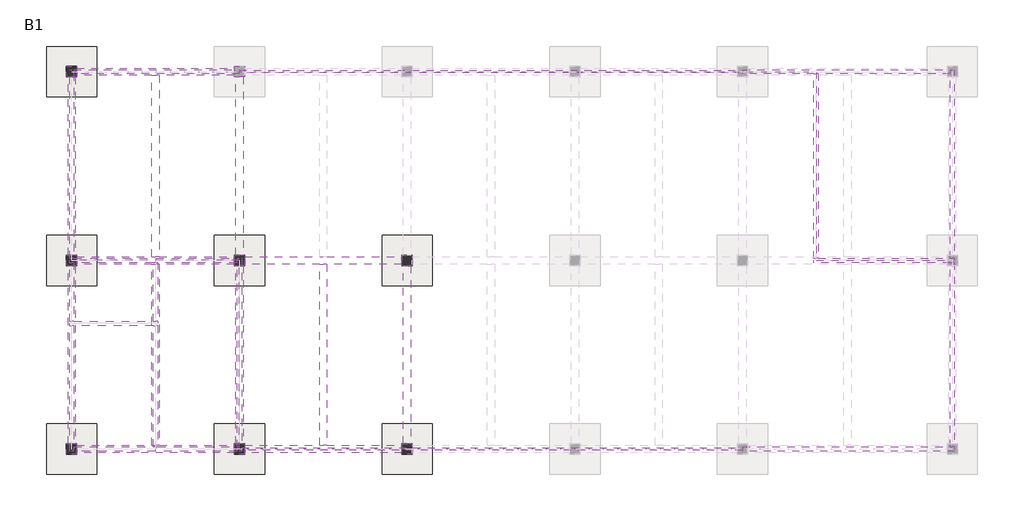
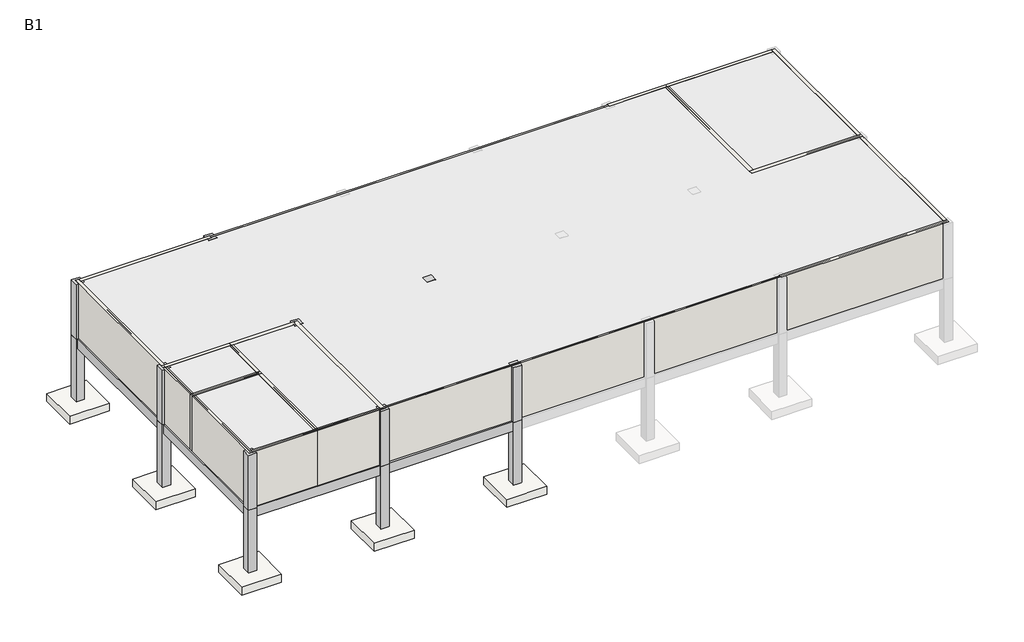
# One storey, part 1 of 2: 20 walls, 15 columns, 13 beams, 12 slabs.
"""IFC4 building model written with IfcOpenShell, lengths in millimetres."""

import ifcopenshell
import ifcopenshell.guid

model = None  # the IFC model being written
_history = None  # IfcOwnerHistory: only IFC2X3 demands one
_inside = {}  # id of a spatial element -> (the spatial element, [elements in it])
_under = {}  # id of a project, library or spatial element -> (it, [spatial elements below it])
_declared = {}  # id of a project -> (the project, [libraries it declares])
_typed = {}  # id of a type object -> (the type object, [elements of that type])
_made_of = {}  # id of a material, layer set ... -> (it, [elements and type objects made of it])


def new_model(schema):
    """Start an empty IFC model of exactly this schema.

    Asked for "IFC4X3", IfcOpenShell would pick the latest addendum, in which some entities
    have other attributes; the version numbers below select the first issue.
    IFC2X3 requires an IfcOwnerHistory on every rooted entity: one is made here for all.
    """
    global model, _history
    if schema == "IFC4X3":
        model = ifcopenshell.file(schema_version=(4, 3, 0, 0))
    else:
        model = ifcopenshell.file(schema=schema)
    _inside.clear()
    _under.clear()
    _declared.clear()
    _typed.clear()
    _made_of.clear()
    _history = None
    if model.schema == "IFC2X3":
        org = make("IfcOrganization", Name="unknown")
        user = make(
            "IfcPersonAndOrganization",
            ThePerson=make("IfcPerson", FamilyName="unknown"),
            TheOrganization=org,
        )
        app = make(
            "IfcApplication",
            ApplicationDeveloper=org,
            Version="unknown",
            ApplicationFullName="unknown",
            ApplicationIdentifier="unknown",
        )
        _history = make(
            "IfcOwnerHistory",
            OwningUser=user,
            OwningApplication=app,
            ChangeAction="ADDED",
            CreationDate=0,
        )
    return model


def make(cls, **values):
    """One entity of the class cls with the attributes given. An attribute that is None is left unset."""
    return model.create_entity(
        cls, **{name: value for name, value in values.items() if value is not None}
    )


def rooted(cls, **values):
    """An entity with a GlobalId (a new one), such as an element, a storey or a relation."""
    return make(cls, GlobalId=ifcopenshell.guid.new(), OwnerHistory=_history, **values)


def si_unit(unit_type, name, prefix=None):
    """IfcSIUnit, for example si_unit("LENGTHUNIT", "METRE", prefix="MILLI")."""
    return make("IfcSIUnit", UnitType=unit_type, Prefix=prefix, Name=name)


def assignment(units):
    """IfcUnitAssignment: the units of a project."""
    return None if units is None else make("IfcUnitAssignment", Units=units)


def point(xyz):
    """IfcCartesianPoint."""
    return None if xyz is None else make("IfcCartesianPoint", Coordinates=xyz)


def direction(xyz):
    """IfcDirection."""
    return None if xyz is None else make("IfcDirection", DirectionRatios=xyz)


def frame(location, z_axis=None, x_axis=None):
    """IfcAxis2Placement3D, a coordinate frame: its origin and axes. An axis left out is left unset."""
    return make(
        "IfcAxis2Placement3D",
        Location=point(location),
        Axis=direction(z_axis),
        RefDirection=direction(x_axis),
    )


def origin():
    """The frame at (0, 0, 0) with its axes left unset."""
    return frame((0.0, 0.0, 0.0))


def origin_with_axes():
    """The frame at (0, 0, 0) with the z axis (0, 0, 1) and the x axis (1, 0, 0) written out."""
    return frame((0.0, 0.0, 0.0), z_axis=(0.0, 0.0, 1.0), x_axis=(1.0, 0.0, 0.0))


def place(relative_to, where):
    """IfcLocalPlacement: puts the frame where relative to a parent placement (None: the world)."""
    return make(
        "IfcLocalPlacement", PlacementRelTo=relative_to, RelativePlacement=where
    )


def context(
    kind, dimensions, precision=None, world=None, true_north=None, identifier=None
):
    """IfcGeometricRepresentationContext, for example the 3D "Model" context."""
    return make(
        "IfcGeometricRepresentationContext",
        ContextIdentifier=identifier,
        ContextType=kind,
        CoordinateSpaceDimension=dimensions,
        Precision=precision,
        WorldCoordinateSystem=world,
        TrueNorth=true_north,
    )


def project(units=None, contexts=None):
    """IfcProject with its units and contexts."""
    return rooted(
        "IfcProject",
        Name="project",
        RepresentationContexts=contexts,
        UnitsInContext=assignment(units),
    )


def spatial(cls, under=None, at=None, **own):
    """A site, building, storey or space (cls), placed at a placement, below another one or the project."""
    s = rooted(cls, ObjectPlacement=at, **own)
    if under is not None:
        _under.setdefault(under.id(), (under, []))[1].append(s)
    return s


def polyline(points):
    """IfcPolyline through the points."""
    return make("IfcPolyline", Points=[point(p) for p in points])


def outline(outer, holes=None, kind="AREA"):
    """IfcArbitraryClosedProfileDef: a profile drawn as a closed curve; with holes, ...WithVoids."""
    if holes is None:
        return make("IfcArbitraryClosedProfileDef", ProfileType=kind, OuterCurve=outer)
    return make(
        "IfcArbitraryProfileDefWithVoids",
        ProfileType=kind,
        OuterCurve=outer,
        InnerCurves=holes,
    )


def extrude(swept, where, along, depth):
    """IfcExtrudedAreaSolid: the profile swept, set in the frame where, extruded along a direction by depth."""
    return make(
        "IfcExtrudedAreaSolid",
        SweptArea=swept,
        Position=where,
        ExtrudedDirection=direction(along),
        Depth=depth,
    )


def faces_of(points, faces, orient=None, outer=None):
    """IfcFace entities. A face is a list of loops; a loop is a list of indices into points, from 0.

    orient and outer hold one flag for each loop. By default every Orientation is true, the
    first loop of a face is its IfcFaceOuterBound and the others are IfcFaceBound.
    """
    made = []
    for i, loops in enumerate(faces):
        bounds = []
        for j, loop in enumerate(loops):
            is_outer = j == 0 if outer is None else outer[i][j]
            bounds.append(
                make(
                    "IfcFaceOuterBound" if is_outer else "IfcFaceBound",
                    Bound=make("IfcPolyLoop", Polygon=[points[k] for k in loop]),
                    Orientation=True if orient is None else orient[i][j],
                )
            )
        made.append(make("IfcFace", Bounds=bounds))
    return made


def faceted_brep(points, faces, orient=None, outer=None, voids=None):
    """IfcFacetedBrep: a solid bounded by flat faces; with voids (closed shells), ...WithVoids."""
    shared = [point(p) for p in points]
    hull = make("IfcClosedShell", CfsFaces=faces_of(shared, faces, orient, outer))
    if voids is None:
        return make("IfcFacetedBrep", Outer=hull)
    return make(
        "IfcFacetedBrepWithVoids",
        Outer=hull,
        Voids=[
            make(cls, CfsFaces=faces_of(shared, fs, o, b)) for cls, fs, o, b in voids
        ],
    )


def shape(context_of_items, identifier, shape_type, items):
    """IfcShapeRepresentation: the items that make up one representation, for example the "Body"."""
    return make(
        "IfcShapeRepresentation",
        ContextOfItems=context_of_items,
        RepresentationIdentifier=identifier,
        RepresentationType=shape_type,
        Items=items,
    )


def source(mapping_origin, context_of_items, identifier, shape_type, items):
    """IfcRepresentationMap: a shape defined once, which mapped items show again and again."""
    return make(
        "IfcRepresentationMap",
        MappingOrigin=mapping_origin,
        MappedRepresentation=shape(context_of_items, identifier, shape_type, items),
    )


def transform(
    local_origin,
    x_axis=None,
    y_axis=None,
    z_axis=None,
    scale=None,
    scale2=None,
    scale3=None,
    uniform=True,
):
    """IfcCartesianTransformationOperator3D, or its non-uniform kind. x_axis, y_axis, z_axis: its Axis1, 2, 3."""
    if uniform:
        return make(
            "IfcCartesianTransformationOperator3D",
            Axis1=direction(x_axis),
            Axis2=direction(y_axis),
            LocalOrigin=point(local_origin),
            Scale=scale,
            Axis3=direction(z_axis),
        )
    return make(
        "IfcCartesianTransformationOperator3DnonUniform",
        Axis1=direction(x_axis),
        Axis2=direction(y_axis),
        LocalOrigin=point(local_origin),
        Scale=scale,
        Axis3=direction(z_axis),
        Scale2=scale2,
        Scale3=scale3,
    )


def mapped(mapping_source, mapping_target):
    """IfcMappedItem: shows the shape of a source again, moved by a transform."""
    return make(
        "IfcMappedItem", MappingSource=mapping_source, MappingTarget=mapping_target
    )


def made_of(thing, what):
    """Note that an element or type object is made of a material, layer set ...; save() writes the relation."""
    if what is not None:
        _made_of.setdefault(what.id(), (what, []))[1].append(thing)
    return thing


def element(
    cls,
    number,
    at=None,
    inside=None,
    cuts=None,
    type_object=None,
    material=None,
    context=None,
    identifier="Body",
    shape_type=None,
    held_by="IfcProductDefinitionShape",
    body=None,
    shapes=None,
    **own,
):
    """One element of the class cls, such as IfcWall. Its Tag is "e" and its number.

    at: its placement. inside: the storey or other place that contains it. cuts: it is an
    opening in that element (IfcRelVoidsElement). A single representation is given by context,
    identifier, shape_type and body (its items); several are given by shapes. held_by: the class
    of the entity that holds the representations. save() writes the other relations.
    """
    e = rooted(cls, Tag="e%d" % number, ObjectPlacement=at, **own)
    if body is not None:
        shapes = [shape(context, identifier, shape_type, body)]
    if shapes is not None:
        e.Representation = make(held_by, Representations=shapes)
    if inside is not None:
        _inside.setdefault(inside.id(), (inside, []))[1].append(e)
    if cuts is not None:
        rooted(
            "IfcRelVoidsElement", RelatingBuildingElement=cuts, RelatedOpeningElement=e
        )
    if type_object is not None:
        _typed.setdefault(type_object.id(), (type_object, []))[1].append(e)
    return made_of(e, material)


def aggregate(whole, parts):
    """IfcRelAggregates: a whole, such as a stair, and the parts it consists of."""
    return rooted("IfcRelAggregates", RelatingObject=whole, RelatedObjects=parts)


def save(model, path):
    """Write the relations noted so far, then the file.

    IfcRelAggregates (storeys below a building ...), IfcRelContainedInSpatialStructure (elements
    in a storey), IfcRelDefinesByType, IfcRelAssociatesMaterial and IfcRelDeclares: one each for
    every whole, place, type object, material and project.
    """
    for whole, parts in _under.values():
        aggregate(whole, parts)
    for where, things in _inside.values():
        rooted(
            "IfcRelContainedInSpatialStructure",
            RelatedElements=things,
            RelatingStructure=where,
        )
    for kind, things in _typed.values():
        rooted("IfcRelDefinesByType", RelatedObjects=things, RelatingType=kind)
    for what, things in _made_of.values():
        rooted("IfcRelAssociatesMaterial", RelatedObjects=things, RelatingMaterial=what)
    for by, libraries in _declared.values():
        rooted("IfcRelDeclares", RelatingContext=by, RelatedDefinitions=libraries)
    model.write(path)


def ft112_footing_rectangular_ft112_2400x2400x500_5fe39465(model_context):
    return source(origin(), model_context, "Body", "SweptSolid", [
        extrude(outline(polyline([(1200.0, 1200.0), (1200.0, -1200.0), (-1200.0, -1200.0), (-1200.0, 1200.0), (1200.0, 1200.0)])), frame((0.0, 0.0, -500.0), z_axis=(0.0, 0.0, 1.0), x_axis=(1.0, 0.0, 0.0)), (0.0, 0.0, 1.0), 500.0),
    ])


model = new_model("IFC4")

# Units and contexts
model_context = context("Model", 3, world=origin())
ifc_project = project(units=[si_unit("LENGTHUNIT", "METRE", prefix="MILLI")], contexts=[model_context])

# Site, building, storey
site = spatial("IfcSite", under=ifc_project)
building = spatial("IfcBuilding", under=site)
storey = spatial("IfcBuildingStorey", under=building, Name="B1", Elevation=-4000.0)

# Beams
placement = place(None, origin())
element("IfcBeam", 1, ObjectType="Concrete-Rectangular-Beam : BM111_400x500_RG1", at=placement, inside=storey, context=model_context, shape_type="SweptSolid", body=[
    extrude(outline(polyline([(49284.6521483, 181748.8614395), (49634.6521483, 181748.8614395), (49634.6521483, 173098.8614395), (49284.6521483, 173098.8614395), (49284.6521483, 181748.8614395)])), frame((0.0, 0.0, -600.0), z_axis=(0.0, 0.0, 1.0), x_axis=(1.0, 0.0, 0.0)), (0.0, 0.0, 1.0), 600.0),
])
element("IfcBeam", 2, ObjectType="Concrete-Rectangular-Beam : BM111_400x500_RG1", at=placement, inside=storey, context=model_context, shape_type="SweptSolid", body=[
    extrude(outline(polyline([(49284.6521483, 172748.8614395), (49634.6521483, 172748.8614395), (49634.6521483, 164098.8614395), (49284.6521483, 164098.8614395), (49284.6521483, 172748.8614395)])), frame((0.0, 0.0, -600.0), z_axis=(0.0, 0.0, 1.0), x_axis=(1.0, 0.0, 0.0)), (0.0, 0.0, 1.0), 600.0),
])
element("IfcBeam", 3, ObjectType="Concrete-Rectangular-Beam : BM111_400x500_RG1", at=placement, inside=storey, context=model_context, shape_type="SweptSolid", body=[
    extrude(outline(polyline([(57284.6521483, 172748.8614395), (57634.6521483, 172748.8614395), (57634.6521483, 164098.8614395), (57284.6521483, 164098.8614395), (57284.6521483, 172748.8614395)])), frame((0.0, 0.0, -600.0), z_axis=(0.0, 0.0, 1.0), x_axis=(1.0, 0.0, 0.0)), (0.0, 0.0, 1.0), 600.0),
])
element("IfcBeam", 4, ObjectType="Concrete-Rectangular-Beam : BM111_400x500_RG1", at=placement, inside=storey, context=model_context, shape_type="Brep", body=[
    faceted_brep([(45709.6521483, 182098.8614395, 0.0), (45709.6521483, 181748.8614395, 0.0), (49284.6521483, 181748.8614395, 0.0), (49634.6521483, 181748.8614395, 0.0), (53209.6521483, 181748.8614395, 0.0), (53209.6521483, 182098.8614395, 0.0), (45709.6521483, 181748.8614395, -600.0), (49284.6521483, 181748.8614395, -600.0), (49634.6521483, 181748.8614395, -600.0), (53209.6521483, 181748.8614395, -600.0), (45709.6521483, 182098.8614395, -600.0), (53209.6521483, 182098.8614395, -600.0)], [[[0, 1, 2, 3, 4, 5]], [[1, 6, 7, 8, 9, 4, 3, 2]], [[6, 10, 11, 9, 8, 7]], [[10, 0, 5, 11]], [[1, 0, 10, 6]], [[5, 4, 9, 11]]]),
])
element("IfcBeam", 5, ObjectType="Concrete-Rectangular-Beam : BM111_400x500_RG1", at=placement, inside=storey, context=model_context, shape_type="Brep", body=[
    faceted_brep([(45709.6521483, 173098.8614395, 0.0), (45709.6521483, 172748.8614395, 0.0), (49284.6521483, 172748.8614395, 0.0), (49634.6521483, 172748.8614395, 0.0), (53209.6521483, 172748.8614395, 0.0), (53209.6521483, 173098.8614395, 0.0), (49634.6521483, 173098.8614395, 0.0), (49284.6521483, 173098.8614395, 0.0), (45709.6521483, 172748.8614395, -600.0), (49284.6521483, 172748.8614395, -600.0), (49634.6521483, 172748.8614395, -600.0), (53209.6521483, 172748.8614395, -600.0), (45709.6521483, 173098.8614395, -600.0), (49284.6521483, 173098.8614395, -600.0), (49634.6521483, 173098.8614395, -600.0), (53209.6521483, 173098.8614395, -600.0)], [[[0, 1, 2, 3, 4, 5, 6, 7]], [[1, 8, 9, 10, 11, 4, 3, 2]], [[8, 12, 13, 14, 15, 11, 10, 9]], [[12, 0, 7, 6, 5, 15, 14, 13]], [[1, 0, 12, 8]], [[5, 4, 11, 15]]]),
])
element("IfcBeam", 6, ObjectType="Concrete-Rectangular-Beam : BM111_400x500_RG1", at=placement, inside=storey, context=model_context, shape_type="Brep", body=[
    faceted_brep([(53709.6521483, 173098.8614395, 0.0), (53709.6521483, 172748.8614395, 0.0), (57284.6521483, 172748.8614395, 0.0), (57634.6521483, 172748.8614395, 0.0), (61209.6521483, 172748.8614395, 0.0), (61209.6521483, 173098.8614395, 0.0), (57634.6521483, 173098.8614395, 0.0), (57284.6521483, 173098.8614395, 0.0), (53709.6521483, 172748.8614395, -600.0), (57284.6521483, 172748.8614395, -600.0), (57634.6521483, 172748.8614395, -600.0), (61209.6521483, 172748.8614395, -600.0), (53709.6521483, 173098.8614395, -600.0), (57284.6521483, 173098.8614395, -600.0), (57634.6521483, 173098.8614395, -600.0), (61209.6521483, 173098.8614395, -600.0)], [[[0, 1, 2, 3, 4, 5, 6, 7]], [[1, 8, 9, 10, 11, 4, 3, 2]], [[8, 12, 13, 14, 15, 11, 10, 9]], [[12, 0, 7, 6, 5, 15, 14, 13]], [[1, 0, 12, 8]], [[5, 4, 11, 15]]]),
])
element("IfcBeam", 7, ObjectType="Concrete-Rectangular-Beam : BM111_400x500_RG1", at=placement, inside=storey, context=model_context, shape_type="Brep", body=[
    faceted_brep([(45709.6521483, 164098.8614395, 0.0), (45709.6521483, 163748.8614395, 0.0), (53209.6521483, 163748.8614395, 0.0), (53209.6521483, 164098.8614395, 0.0), (49634.6521483, 164098.8614395, 0.0), (49284.6521483, 164098.8614395, 0.0), (45709.6521483, 163748.8614395, -600.0), (53209.6521483, 163748.8614395, -600.0), (45709.6521483, 164098.8614395, -600.0), (49284.6521483, 164098.8614395, -600.0), (49634.6521483, 164098.8614395, -600.0), (53209.6521483, 164098.8614395, -600.0)], [[[0, 1, 2, 3, 4, 5]], [[1, 6, 7, 2]], [[6, 8, 9, 10, 11, 7]], [[8, 0, 5, 4, 3, 11, 10, 9]], [[1, 0, 8, 6]], [[3, 2, 7, 11]]]),
])
element("IfcBeam", 8, ObjectType="Concrete-Rectangular-Beam : BM111_400x500_RG1", at=placement, inside=storey, context=model_context, shape_type="Brep", body=[
    faceted_brep([(53709.6521483, 164098.8614395, 0.0), (53709.6521483, 163748.8614395, 0.0), (61209.6521483, 163748.8614395, 0.0), (61209.6521483, 164098.8614395, 0.0), (57634.6521483, 164098.8614395, 0.0), (57284.6521483, 164098.8614395, 0.0), (53709.6521483, 163748.8614395, -600.0), (61209.6521483, 163748.8614395, -600.0), (53709.6521483, 164098.8614395, -600.0), (57284.6521483, 164098.8614395, -600.0), (57634.6521483, 164098.8614395, -600.0), (61209.6521483, 164098.8614395, -600.0)], [[[0, 1, 2, 3, 4, 5]], [[1, 6, 7, 2]], [[6, 8, 9, 10, 11, 7]], [[8, 0, 5, 4, 3, 11, 10, 9]], [[1, 0, 8, 6]], [[3, 2, 7, 11]]]),
])
element("IfcBeam", 9, ObjectType="Concrete-Rectangular-Beam : BM111_400x500_RG1", at=placement, inside=storey, context=model_context, shape_type="SweptSolid", body=[
    extrude(outline(polyline([(45284.6521483, 181673.8614395), (45634.6521483, 181673.8614395), (45634.6521483, 173173.8614395), (45284.6521483, 173173.8614395), (45284.6521483, 181673.8614395)])), frame((0.0, 0.0, -600.0), z_axis=(0.0, 0.0, 1.0), x_axis=(1.0, 0.0, 0.0)), (0.0, 0.0, 1.0), 600.0),
])
element("IfcBeam", 10, ObjectType="Concrete-Rectangular-Beam : BM111_400x500_RG1", at=placement, inside=storey, context=model_context, shape_type="SweptSolid", body=[
    extrude(outline(polyline([(45284.6521483, 172673.8614395), (45634.6521483, 172673.8614395), (45634.6521483, 164173.8614395), (45284.6521483, 164173.8614395), (45284.6521483, 172673.8614395)])), frame((0.0, 0.0, -600.0), z_axis=(0.0, 0.0, 1.0), x_axis=(1.0, 0.0, 0.0)), (0.0, 0.0, 1.0), 600.0),
])
element("IfcBeam", 11, ObjectType="Concrete-Rectangular-Beam : BM111_400x500_RG1", at=placement, inside=storey, context=model_context, shape_type="SweptSolid", body=[
    extrude(outline(polyline([(53284.6521483, 181673.8614395), (53634.6521483, 181673.8614395), (53634.6521483, 173173.8614395), (53284.6521483, 173173.8614395), (53284.6521483, 181673.8614395)])), frame((0.0, 0.0, -600.0), z_axis=(0.0, 0.0, 1.0), x_axis=(1.0, 0.0, 0.0)), (0.0, 0.0, 1.0), 600.0),
])
element("IfcBeam", 12, ObjectType="Concrete-Rectangular-Beam : BM111_400x500_RG1", at=placement, inside=storey, context=model_context, shape_type="SweptSolid", body=[
    extrude(outline(polyline([(53284.6521483, 172673.8614395), (53634.6521483, 172673.8614395), (53634.6521483, 164173.8614395), (53284.6521483, 164173.8614395), (53284.6521483, 172673.8614395)])), frame((0.0, 0.0, -600.0), z_axis=(0.0, 0.0, 1.0), x_axis=(1.0, 0.0, 0.0)), (0.0, 0.0, 1.0), 600.0),
])
element("IfcBeam", 13, ObjectType="Concrete-Rectangular-Beam : BM111_400x500_RG1", at=placement, inside=storey, context=model_context, shape_type="SweptSolid", body=[
    extrude(outline(polyline([(61284.6521483, 172673.8614395), (61634.6521483, 172673.8614395), (61634.6521483, 164173.8614395), (61284.6521483, 164173.8614395), (61284.6521483, 172673.8614395)])), frame((0.0, 0.0, -600.0), z_axis=(0.0, 0.0, 1.0), x_axis=(1.0, 0.0, 0.0)), (0.0, 0.0, 1.0), 600.0),
])

# Columns
element("IfcColumn", 14, ObjectType="Concrete-Rectangular-Column : CL111_500x500", at=placement, inside=storey, context=model_context, shape_type="Brep", body=[
    faceted_brep([(45709.6521483, 182173.8614395, 0.0), (45709.6521483, 181673.8614395, 0.0), (45209.6521483, 181673.8614395, 0.0), (45209.6521483, 182173.8614395, 0.0), (45709.6521483, 182173.8614395, 3500.0), (45709.6521483, 182098.8614395, 3500.0), (45709.6521483, 181748.8614395, 3500.0), (45709.6521483, 181673.8614395, 3500.0), (45634.6521483, 181673.8614395, 3500.0), (45284.6521483, 181673.8614395, 3500.0), (45209.6521483, 181673.8614395, 3500.0), (45209.6521483, 182173.8614395, 3500.0)], [[[0, 1, 2, 3]], [[4, 5, 6, 7, 1, 0]], [[7, 8, 9, 10, 2, 1]], [[10, 11, 3, 2]], [[11, 4, 0, 3]], [[4, 11, 10, 9, 8, 7, 6, 5]]]),
])
element("IfcColumn", 15, ObjectType="Concrete-Rectangular-Column : CL111_500x500", at=placement, inside=storey, context=model_context, shape_type="Brep", body=[
    faceted_brep([(53709.6521483, 182173.8614395, 0.0), (53709.6521483, 181673.8614395, 0.0), (53209.6521483, 181673.8614395, 0.0), (53209.6521483, 182173.8614395, 0.0), (53709.6521483, 182173.8614395, 3500.0), (53709.6521483, 182098.8614395, 3500.0), (53709.6521483, 181748.8614395, 3500.0), (53709.6521483, 181673.8614395, 3500.0), (53634.6521483, 181673.8614395, 3500.0), (53284.6521483, 181673.8614395, 3500.0), (53209.6521483, 181673.8614395, 3500.0), (53209.6521483, 181748.8614395, 3500.0), (53209.6521483, 182098.8614395, 3500.0), (53209.6521483, 182173.8614395, 3500.0)], [[[0, 1, 2, 3]], [[4, 5, 6, 7, 1, 0]], [[7, 8, 9, 10, 2, 1]], [[10, 11, 12, 13, 3, 2]], [[13, 4, 0, 3]], [[4, 13, 12, 11, 10, 9, 8, 7, 6, 5]]]),
])
element("IfcColumn", 16, ObjectType="Concrete-Rectangular-Column : CL111_500x500", at=placement, inside=storey, context=model_context, shape_type="Brep", body=[
    faceted_brep([(45709.6521483, 173173.8614395, 0.0), (45709.6521483, 172673.8614395, 0.0), (45209.6521483, 172673.8614395, 0.0), (45209.6521483, 173173.8614395, 0.0), (45709.6521483, 173173.8614395, 3500.0), (45709.6521483, 173098.8614395, 3500.0), (45709.6521483, 172748.8614395, 3500.0), (45709.6521483, 172673.8614395, 3500.0), (45634.6521483, 172673.8614395, 3500.0), (45284.6521483, 172673.8614395, 3500.0), (45209.6521483, 172673.8614395, 3500.0), (45209.6521483, 173173.8614395, 3500.0), (45284.6521483, 173173.8614395, 3500.0), (45634.6521483, 173173.8614395, 3500.0)], [[[0, 1, 2, 3]], [[4, 5, 6, 7, 1, 0]], [[7, 8, 9, 10, 2, 1]], [[10, 11, 3, 2]], [[11, 12, 13, 4, 0, 3]], [[4, 13, 12, 11, 10, 9, 8, 7, 6, 5]]]),
])
element("IfcColumn", 17, ObjectType="Concrete-Rectangular-Column : CL111_500x500", at=placement, inside=storey, context=model_context, shape_type="Brep", body=[
    faceted_brep([(53709.6521483, 173173.8614395, 0.0), (53709.6521483, 172673.8614395, 0.0), (53209.6521483, 172673.8614395, 0.0), (53209.6521483, 173173.8614395, 0.0), (53709.6521483, 173173.8614395, 3500.0), (53709.6521483, 173098.8614395, 3500.0), (53709.6521483, 172748.8614395, 3500.0), (53709.6521483, 172673.8614395, 3500.0), (53634.6521483, 172673.8614395, 3500.0), (53284.6521483, 172673.8614395, 3500.0), (53209.6521483, 172673.8614395, 3500.0), (53209.6521483, 172748.8614395, 3500.0), (53209.6521483, 173098.8614395, 3500.0), (53209.6521483, 173173.8614395, 3500.0), (53284.6521483, 173173.8614395, 3500.0), (53634.6521483, 173173.8614395, 3500.0)], [[[0, 1, 2, 3]], [[4, 5, 6, 7, 1, 0]], [[7, 8, 9, 10, 2, 1]], [[10, 11, 12, 13, 3, 2]], [[13, 14, 15, 4, 0, 3]], [[4, 15, 14, 13, 12, 11, 10, 9, 8, 7, 6, 5]]]),
])
element("IfcColumn", 18, ObjectType="Concrete-Rectangular-Column : CL111_500x500", at=placement, inside=storey, context=model_context, shape_type="Brep", body=[
    faceted_brep([(61709.6521483, 173173.8614395, 0.0), (61709.6521483, 172673.8614395, 0.0), (61209.6521483, 172673.8614395, 0.0), (61209.6521483, 173173.8614395, 0.0), (61709.6521483, 173173.8614395, 3500.0), (61709.6521483, 173098.8614395, 3500.0), (61709.6521483, 172748.8614395, 3500.0), (61709.6521483, 172673.8614395, 3500.0), (61634.6521483, 172673.8614395, 3500.0), (61284.6521483, 172673.8614395, 3500.0), (61209.6521483, 172673.8614395, 3500.0), (61209.6521483, 172748.8614395, 3500.0), (61209.6521483, 173098.8614395, 3500.0), (61209.6521483, 173173.8614395, 3500.0), (61284.6521483, 173173.8614395, 3500.0), (61634.6521483, 173173.8614395, 3500.0)], [[[0, 1, 2, 3]], [[4, 5, 6, 7, 1, 0]], [[7, 8, 9, 10, 2, 1]], [[10, 11, 12, 13, 3, 2]], [[13, 14, 15, 4, 0, 3]], [[4, 15, 14, 13, 12, 11, 10, 9, 8, 7, 6, 5]]]),
])
element("IfcColumn", 19, ObjectType="Concrete-Rectangular-Column : CL111_500x500", at=placement, inside=storey, context=model_context, shape_type="Brep", body=[
    faceted_brep([(45709.6521483, 164173.8614395, 0.0), (45709.6521483, 163673.8614395, 0.0), (45209.6521483, 163673.8614395, 0.0), (45209.6521483, 164173.8614395, 0.0), (45709.6521483, 164173.8614395, 3500.0), (45709.6521483, 164098.8614395, 3500.0), (45709.6521483, 163748.8614395, 3500.0), (45709.6521483, 163673.8614395, 3500.0), (45209.6521483, 163673.8614395, 3500.0), (45209.6521483, 164173.8614395, 3500.0), (45284.6521483, 164173.8614395, 3500.0), (45634.6521483, 164173.8614395, 3500.0)], [[[0, 1, 2, 3]], [[4, 5, 6, 7, 1, 0]], [[7, 8, 2, 1]], [[8, 9, 3, 2]], [[9, 10, 11, 4, 0, 3]], [[4, 11, 10, 9, 8, 7, 6, 5]]]),
])
element("IfcColumn", 20, ObjectType="Concrete-Rectangular-Column : CL111_500x500", at=placement, inside=storey, context=model_context, shape_type="Brep", body=[
    faceted_brep([(53709.6521483, 164173.8614395, 0.0), (53709.6521483, 163673.8614395, 0.0), (53209.6521483, 163673.8614395, 0.0), (53209.6521483, 164173.8614395, 0.0), (53709.6521483, 164173.8614395, 3500.0), (53709.6521483, 164098.8614395, 3500.0), (53709.6521483, 163748.8614395, 3500.0), (53709.6521483, 163673.8614395, 3500.0), (53209.6521483, 163673.8614395, 3500.0), (53209.6521483, 163748.8614395, 3500.0), (53209.6521483, 164098.8614395, 3500.0), (53209.6521483, 164173.8614395, 3500.0), (53284.6521483, 164173.8614395, 3500.0), (53634.6521483, 164173.8614395, 3500.0)], [[[0, 1, 2, 3]], [[4, 5, 6, 7, 1, 0]], [[7, 8, 2, 1]], [[8, 9, 10, 11, 3, 2]], [[11, 12, 13, 4, 0, 3]], [[4, 13, 12, 11, 10, 9, 8, 7, 6, 5]]]),
])
element("IfcColumn", 21, ObjectType="Concrete-Rectangular-Column : CL111_500x500", at=placement, inside=storey, context=model_context, shape_type="Brep", body=[
    faceted_brep([(61709.6521483, 164173.8614395, 0.0), (61709.6521483, 163673.8614395, 0.0), (61209.6521483, 163673.8614395, 0.0), (61209.6521483, 164173.8614395, 0.0), (61709.6521483, 164173.8614395, 3500.0), (61709.6521483, 164098.8614395, 3500.0), (61709.6521483, 163748.8614395, 3500.0), (61709.6521483, 163673.8614395, 3500.0), (61209.6521483, 163673.8614395, 3500.0), (61209.6521483, 163748.8614395, 3500.0), (61209.6521483, 164098.8614395, 3500.0), (61209.6521483, 164173.8614395, 3500.0), (61284.6521483, 164173.8614395, 3500.0), (61634.6521483, 164173.8614395, 3500.0)], [[[0, 1, 2, 3]], [[4, 5, 6, 7, 1, 0]], [[7, 8, 2, 1]], [[8, 9, 10, 11, 3, 2]], [[11, 12, 13, 4, 0, 3]], [[4, 13, 12, 11, 10, 9, 8, 7, 6, 5]]]),
])
element("IfcColumn", 22, ObjectType="Concrete-Rectangular-Column : CL111_500x500", at=placement, inside=storey, context=model_context, shape_type="Brep", body=[
    faceted_brep([(45709.6521483, 182173.8614395, -4000.0), (45709.6521483, 181673.8614395, -4000.0), (45209.6521483, 181673.8614395, -4000.0), (45209.6521483, 182173.8614395, -4000.0), (45709.6521483, 182173.8614395, 0.0), (45709.6521483, 182098.8614395, 0.0), (45709.6521483, 181748.8614395, 0.0), (45709.6521483, 181673.8614395, 0.0), (45634.6521483, 181673.8614395, 0.0), (45284.6521483, 181673.8614395, 0.0), (45209.6521483, 181673.8614395, 0.0), (45209.6521483, 182173.8614395, 0.0)], [[[0, 1, 2, 3]], [[4, 5, 6, 7, 1, 0]], [[7, 8, 9, 10, 2, 1]], [[10, 11, 3, 2]], [[11, 4, 0, 3]], [[4, 11, 10, 9, 8, 7, 6, 5]]]),
])
element("IfcColumn", 23, ObjectType="Concrete-Rectangular-Column : CL111_500x500", at=placement, inside=storey, context=model_context, shape_type="Brep", body=[
    faceted_brep([(45709.6521483, 173173.8614395, -4000.0), (45709.6521483, 172673.8614395, -4000.0), (45209.6521483, 172673.8614395, -4000.0), (45209.6521483, 173173.8614395, -4000.0), (45709.6521483, 173173.8614395, 0.0), (45709.6521483, 173098.8614395, 0.0), (45709.6521483, 172748.8614395, 0.0), (45709.6521483, 172673.8614395, 0.0), (45634.6521483, 172673.8614395, 0.0), (45284.6521483, 172673.8614395, 0.0), (45209.6521483, 172673.8614395, 0.0), (45209.6521483, 173173.8614395, 0.0), (45284.6521483, 173173.8614395, 0.0), (45634.6521483, 173173.8614395, 0.0)], [[[0, 1, 2, 3]], [[4, 5, 6, 7, 1, 0]], [[7, 8, 9, 10, 2, 1]], [[10, 11, 3, 2]], [[11, 12, 13, 4, 0, 3]], [[4, 13, 12, 11, 10, 9, 8, 7, 6, 5]]]),
])
element("IfcColumn", 24, ObjectType="Concrete-Rectangular-Column : CL111_500x500", at=placement, inside=storey, context=model_context, shape_type="Brep", body=[
    faceted_brep([(53709.6521483, 173173.8614395, -4000.0), (53709.6521483, 172673.8614395, -4000.0), (53209.6521483, 172673.8614395, -4000.0), (53209.6521483, 173173.8614395, -4000.0), (53709.6521483, 173173.8614395, 0.0), (53709.6521483, 173098.8614395, 0.0), (53709.6521483, 172748.8614395, 0.0), (53709.6521483, 172673.8614395, 0.0), (53634.6521483, 172673.8614395, 0.0), (53284.6521483, 172673.8614395, 0.0), (53209.6521483, 172673.8614395, 0.0), (53209.6521483, 172748.8614395, 0.0), (53209.6521483, 173098.8614395, 0.0), (53209.6521483, 173173.8614395, 0.0), (53284.6521483, 173173.8614395, 0.0), (53634.6521483, 173173.8614395, 0.0)], [[[0, 1, 2, 3]], [[4, 5, 6, 7, 1, 0]], [[7, 8, 9, 10, 2, 1]], [[10, 11, 12, 13, 3, 2]], [[13, 14, 15, 4, 0, 3]], [[4, 15, 14, 13, 12, 11, 10, 9, 8, 7, 6, 5]]]),
])
element("IfcColumn", 25, ObjectType="Concrete-Rectangular-Column : CL111_500x500", at=placement, inside=storey, context=model_context, shape_type="Brep", body=[
    faceted_brep([(61709.6521483, 173173.8614395, -4000.0), (61709.6521483, 172673.8614395, -4000.0), (61209.6521483, 172673.8614395, -4000.0), (61209.6521483, 173173.8614395, -4000.0), (61709.6521483, 173173.8614395, 0.0), (61709.6521483, 173098.8614395, 0.0), (61709.6521483, 172748.8614395, 0.0), (61709.6521483, 172673.8614395, 0.0), (61634.6521483, 172673.8614395, 0.0), (61284.6521483, 172673.8614395, 0.0), (61209.6521483, 172673.8614395, 0.0), (61209.6521483, 172748.8614395, 0.0), (61209.6521483, 173098.8614395, 0.0), (61209.6521483, 173173.8614395, 0.0), (61284.6521483, 173173.8614395, 0.0), (61634.6521483, 173173.8614395, 0.0)], [[[0, 1, 2, 3]], [[4, 5, 6, 7, 1, 0]], [[7, 8, 9, 10, 2, 1]], [[10, 11, 12, 13, 3, 2]], [[13, 14, 15, 4, 0, 3]], [[4, 15, 14, 13, 12, 11, 10, 9, 8, 7, 6, 5]]]),
])
element("IfcColumn", 26, ObjectType="Concrete-Rectangular-Column : CL111_500x500", at=placement, inside=storey, context=model_context, shape_type="Brep", body=[
    faceted_brep([(45709.6521483, 164173.8614395, -4000.0), (45709.6521483, 163673.8614395, -4000.0), (45209.6521483, 163673.8614395, -4000.0), (45209.6521483, 164173.8614395, -4000.0), (45709.6521483, 164173.8614395, 0.0), (45709.6521483, 164098.8614395, 0.0), (45709.6521483, 163748.8614395, 0.0), (45709.6521483, 163673.8614395, 0.0), (45209.6521483, 163673.8614395, 0.0), (45209.6521483, 164173.8614395, 0.0), (45284.6521483, 164173.8614395, 0.0), (45634.6521483, 164173.8614395, 0.0)], [[[0, 1, 2, 3]], [[4, 5, 6, 7, 1, 0]], [[7, 8, 2, 1]], [[8, 9, 3, 2]], [[9, 10, 11, 4, 0, 3]], [[4, 11, 10, 9, 8, 7, 6, 5]]]),
])
element("IfcColumn", 27, ObjectType="Concrete-Rectangular-Column : CL111_500x500", at=placement, inside=storey, context=model_context, shape_type="Brep", body=[
    faceted_brep([(53709.6521483, 164173.8614395, -4000.0), (53709.6521483, 163673.8614395, -4000.0), (53209.6521483, 163673.8614395, -4000.0), (53209.6521483, 164173.8614395, -4000.0), (53709.6521483, 164173.8614395, 0.0), (53709.6521483, 164098.8614395, 0.0), (53709.6521483, 163748.8614395, 0.0), (53709.6521483, 163673.8614395, 0.0), (53209.6521483, 163673.8614395, 0.0), (53209.6521483, 163748.8614395, 0.0), (53209.6521483, 164098.8614395, 0.0), (53209.6521483, 164173.8614395, 0.0), (53284.6521483, 164173.8614395, 0.0), (53634.6521483, 164173.8614395, 0.0)], [[[0, 1, 2, 3]], [[4, 5, 6, 7, 1, 0]], [[7, 8, 2, 1]], [[8, 9, 10, 11, 3, 2]], [[11, 12, 13, 4, 0, 3]], [[4, 13, 12, 11, 10, 9, 8, 7, 6, 5]]]),
])
element("IfcColumn", 28, ObjectType="Concrete-Rectangular-Column : CL111_500x500", at=placement, inside=storey, context=model_context, shape_type="Brep", body=[
    faceted_brep([(61709.6521483, 164173.8614395, -4000.0), (61709.6521483, 163673.8614395, -4000.0), (61209.6521483, 163673.8614395, -4000.0), (61209.6521483, 164173.8614395, -4000.0), (61709.6521483, 164173.8614395, 0.0), (61709.6521483, 164098.8614395, 0.0), (61709.6521483, 163748.8614395, 0.0), (61709.6521483, 163673.8614395, 0.0), (61209.6521483, 163673.8614395, 0.0), (61209.6521483, 163748.8614395, 0.0), (61209.6521483, 164098.8614395, 0.0), (61209.6521483, 164173.8614395, 0.0), (61284.6521483, 164173.8614395, 0.0), (61634.6521483, 164173.8614395, 0.0)], [[[0, 1, 2, 3]], [[4, 5, 6, 7, 1, 0]], [[7, 8, 2, 1]], [[8, 9, 10, 11, 3, 2]], [[11, 12, 13, 4, 0, 3]], [[4, 13, 12, 11, 10, 9, 8, 7, 6, 5]]]),
])

# Slabs
element("IfcSlab", 29, ObjectType="CFS11_Slab RC_T150", at=placement, inside=storey, context=model_context, shape_type="SweptSolid", body=[
    extrude(outline(polyline([(87459.6521483, 181923.8614395), (87459.6521483, 172923.8614395), (80959.6521483, 172923.8614395), (80959.6521483, 181923.8614395), (87459.6521483, 181923.8614395)])), frame((0.0, 0.0, -150.0), z_axis=(0.0, 0.0, 1.0), x_axis=(1.0, 0.0, 0.0)), (0.0, 0.0, 1.0), 150.0),
])
element("IfcSlab", 30, ObjectType="CFS11_Slab RC_T150", at=placement, inside=storey, context=model_context, shape_type="SweptSolid", body=[
    extrude(outline(polyline([(53459.6521483, 163923.8614395), (49459.6521483, 163923.8614395), (49459.6521483, 172923.8614395), (53459.6521483, 172923.8614395), (53459.6521483, 163923.8614395)])), frame((0.0, 0.0, -150.0), z_axis=(0.0, 0.0, 1.0), x_axis=(1.0, 0.0, 0.0)), (0.0, 0.0, 1.0), 150.0),
])
element("IfcSlab", 31, ObjectType="CFS11_Slab RC_T150", at=placement, inside=storey, context=model_context, shape_type="SweptSolid", body=[
    extrude(outline(polyline([(80959.6521483, 181923.8614395), (80959.6521483, 172923.8614395), (87459.6521483, 172923.8614395), (87459.6521483, 163923.8614395), (53459.6521483, 163923.8614395), (53459.6521483, 172923.8614395), (45459.6521483, 172923.8614395), (45459.6521483, 181923.8614395), (80959.6521483, 181923.8614395)])), frame((0.0, 0.0, -150.0), z_axis=(0.0, 0.0, 1.0), x_axis=(1.0, 0.0, 0.0)), (0.0, 0.0, 1.0), 150.0),
])
element("IfcSlab", 32, ObjectType="CFS11_Slab RC_T150", at=placement, inside=storey, context=model_context, shape_type="SweptSolid", body=[
    extrude(outline(polyline([(45459.6521483, 163923.8614395), (45459.6521483, 169923.8614395), (49459.6521483, 169923.8614395), (49459.6521483, 163923.8614395), (45459.6521483, 163923.8614395)])), frame((0.0, 0.0, -150.0), z_axis=(0.0, 0.0, 1.0), x_axis=(1.0, 0.0, 0.0)), (0.0, 0.0, 1.0), 150.0),
])
element("IfcSlab", 33, ObjectType="CFS11_Slab RC_T150", at=placement, inside=storey, context=model_context, shape_type="SweptSolid", body=[
    extrude(outline(polyline([(45459.6521483, 172923.8614395), (49459.6521483, 172923.8614395), (49459.6521483, 169923.8614395), (45459.6521483, 169923.8614395), (45459.6521483, 172923.8614395)])), frame((0.0, 0.0, -150.0), z_axis=(0.0, 0.0, 1.0), x_axis=(1.0, 0.0, 0.0)), (0.0, 0.0, 1.0), 150.0),
])
ft112_footing_rectangular_ft112_2400x2400x500_shape = ft112_footing_rectangular_ft112_2400x2400x500_5fe39465(model_context)
element("IfcSlab", 34, ObjectType="FT112-Footing-Rectangular : FT112_2400x2400x500", at=placement, inside=storey, context=model_context, shape_type="MappedRepresentation", body=[
    mapped(ft112_footing_rectangular_ft112_2400x2400x500_shape, transform((45459.6521483, 181923.8614395, -4000.0), x_axis=(1.0, 0.0, 0.0), y_axis=(0.0, 1.0, 0.0), z_axis=(0.0, 0.0, 1.0))),
])
element("IfcSlab", 35, ObjectType="FT112-Footing-Rectangular : FT112_2400x2400x500", at=placement, inside=storey, context=model_context, shape_type="MappedRepresentation", body=[
    mapped(ft112_footing_rectangular_ft112_2400x2400x500_shape, transform((45459.6521483, 172923.8614395, -4000.0), x_axis=(1.0, 0.0, 0.0), y_axis=(0.0, 1.0, 0.0), z_axis=(0.0, 0.0, 1.0))),
])
element("IfcSlab", 36, ObjectType="FT112-Footing-Rectangular : FT112_2400x2400x500", at=placement, inside=storey, context=model_context, shape_type="MappedRepresentation", body=[
    mapped(ft112_footing_rectangular_ft112_2400x2400x500_shape, transform((53459.6521483, 172923.8614395, -4000.0), x_axis=(1.0, 0.0, 0.0), y_axis=(0.0, 1.0, 0.0), z_axis=(0.0, 0.0, 1.0))),
])
element("IfcSlab", 37, ObjectType="FT112-Footing-Rectangular : FT112_2400x2400x500", at=placement, inside=storey, context=model_context, shape_type="MappedRepresentation", body=[
    mapped(ft112_footing_rectangular_ft112_2400x2400x500_shape, transform((61459.6521483, 172923.8614395, -4000.0), x_axis=(1.0, 0.0, 0.0), y_axis=(0.0, 1.0, 0.0), z_axis=(0.0, 0.0, 1.0))),
])
element("IfcSlab", 38, ObjectType="FT112-Footing-Rectangular : FT112_2400x2400x500", at=placement, inside=storey, context=model_context, shape_type="MappedRepresentation", body=[
    mapped(ft112_footing_rectangular_ft112_2400x2400x500_shape, transform((45459.6521483, 163923.8614395, -4000.0), x_axis=(1.0, 0.0, 0.0), y_axis=(0.0, 1.0, 0.0), z_axis=(0.0, 0.0, 1.0))),
])
element("IfcSlab", 39, ObjectType="FT112-Footing-Rectangular : FT112_2400x2400x500", at=placement, inside=storey, context=model_context, shape_type="MappedRepresentation", body=[
    mapped(ft112_footing_rectangular_ft112_2400x2400x500_shape, transform((53459.6521483, 163923.8614395, -4000.0), x_axis=(1.0, 0.0, 0.0), y_axis=(0.0, 1.0, 0.0), z_axis=(0.0, 0.0, 1.0))),
])
element("IfcSlab", 40, ObjectType="FT112-Footing-Rectangular : FT112_2400x2400x500", at=placement, inside=storey, context=model_context, shape_type="MappedRepresentation", body=[
    mapped(ft112_footing_rectangular_ft112_2400x2400x500_shape, transform((61459.6521483, 163923.8614395, -4000.0), x_axis=(1.0, 0.0, 0.0), y_axis=(0.0, 1.0, 0.0), z_axis=(0.0, 0.0, 1.0))),
])

# Walls
element("IfcWall", 41, ObjectType="WA111-Exterior RC Wall 200mm", at=placement, inside=storey, context=model_context, shape_type="Brep", body=[
    faceted_brep([(45559.6521483, 181823.8614395, 0.0), (53459.6521483, 181823.8614395, 0.0), (53459.6521483, 181823.8614395, 3500.0), (45559.6521483, 181823.8614395, 3500.0), (45559.6521483, 182023.8614395, 0.0), (45559.6521483, 182023.8614395, 3500.0), (53459.6521483, 182023.8614395, 3500.0), (53459.6521483, 182023.8614395, 0.0), (53459.6521483, 181980.8614395, 0.0), (53459.6521483, 181866.8614395, 0.0), (53459.6521483, 181980.8614395, 3500.0), (53459.6521483, 181866.8614395, 3500.0)], [[[0, 1, 2, 3]], [[4, 5, 6, 7]], [[1, 0, 4, 7, 8, 9]], [[2, 1, 9, 8, 7, 6, 10, 11]], [[3, 2, 11, 10, 6, 5]], [[0, 3, 5, 4]]]),
])
element("IfcWall", 42, ObjectType="WA111-Exterior RC Wall 200mm", at=placement, inside=storey, context=model_context, shape_type="Brep", body=[
    faceted_brep([(87359.6521483, 182023.8614395, 0.0), (87359.6521483, 181823.8614395, 0.0), (87359.6521483, 173030.8614395, 0.0), (87359.6521483, 173030.8614395, 3500.0), (87359.6521483, 181823.8614395, 3500.0), (87359.6521483, 182023.8614395, 3500.0), (87559.6521483, 182023.8614395, 0.0), (87559.6521483, 182023.8614395, 3500.0), (87559.6521483, 173030.8614395, 3500.0), (87559.6521483, 173030.8614395, 0.0)], [[[0, 1, 2, 3, 4, 5]], [[6, 7, 8, 9]], [[2, 1, 0, 6, 9]], [[5, 4, 3, 8, 7]], [[0, 5, 7, 6]], [[3, 2, 9, 8]]]),
])
element("IfcWall", 43, ObjectType="WA111-Exterior RC Wall 200mm", at=placement, inside=storey, context=model_context, shape_type="Brep", body=[
    faceted_brep([(53352.6521483, 164023.8614395, 0.0), (49566.6521483, 164023.8614395, 0.0), (49459.6521483, 164023.8614395, 0.0), (49459.6521483, 164023.8614395, 3500.0), (49566.6521483, 164023.8614395, 3500.0), (53352.6521483, 164023.8614395, 3500.0), (53352.6521483, 163823.8614395, 0.0), (53352.6521483, 163823.8614395, 3500.0), (49459.6521483, 163823.8614395, 3500.0), (49459.6521483, 163823.8614395, 0.0)], [[[0, 1, 2, 3, 4, 5]], [[6, 7, 8, 9]], [[2, 1, 0, 6, 9]], [[3, 2, 9, 8]], [[5, 4, 3, 8, 7]], [[0, 5, 7, 6]]]),
])
element("IfcWall", 44, ObjectType="WA111-Exterior RC Wall 200mm", at=placement, inside=storey, context=model_context, shape_type="Brep", body=[
    faceted_brep([(45559.6521483, 173030.8614395, 0.0), (45559.6521483, 181823.8614395, 0.0), (45559.6521483, 182023.8614395, 0.0), (45559.6521483, 182023.8614395, 3500.0), (45559.6521483, 181823.8614395, 3500.0), (45559.6521483, 173030.8614395, 3500.0), (45359.6521483, 173030.8614395, 0.0), (45359.6521483, 173030.8614395, 3500.0), (45359.6521483, 182023.8614395, 3500.0), (45359.6521483, 182023.8614395, 0.0)], [[[0, 1, 2, 3, 4, 5]], [[6, 7, 8, 9]], [[2, 1, 0, 6, 9]], [[5, 4, 3, 8, 7]], [[3, 2, 9, 8]], [[0, 5, 7, 6]]]),
])
element("IfcWall", 45, ObjectType="WA111-Exterior RC Wall 200mm", at=placement, inside=storey, context=model_context, shape_type="Brep", body=[
    faceted_brep([(87559.6521483, 164023.8614395, 0.0), (87359.6521483, 164023.8614395, 0.0), (77459.6521483, 164023.8614395, 0.0), (77459.6521483, 164023.8614395, 3500.0), (87359.6521483, 164023.8614395, 3500.0), (87559.6521483, 164023.8614395, 3500.0), (87559.6521483, 163823.8614395, 0.0), (87559.6521483, 163823.8614395, 3500.0), (77459.6521483, 163823.8614395, 3500.0), (77459.6521483, 163823.8614395, 0.0), (77459.6521483, 163866.8614395, 0.0), (77459.6521483, 163980.8614395, 0.0), (77459.6521483, 163866.8614395, 3500.0), (77459.6521483, 163980.8614395, 3500.0)], [[[0, 1, 2, 3, 4, 5]], [[6, 7, 8, 9]], [[2, 1, 0, 6, 9, 10, 11]], [[3, 2, 11, 10, 9, 8, 12, 13]], [[5, 4, 3, 13, 12, 8, 7]], [[0, 5, 7, 6]]]),
])
element("IfcWall", 46, ObjectType="WA111-Exterior RC Wall 200mm", at=placement, inside=storey, context=model_context, shape_type="SweptSolid", body=[
    extrude(outline(polyline([(87359.6521483, 164023.8614395), (87359.6521483, 172816.8614395), (87559.6521483, 172816.8614395), (87559.6521483, 164023.8614395), (87359.6521483, 164023.8614395)])), origin_with_axes(), (0.0, 0.0, 1.0), 3500.0),
])
element("IfcWall", 47, ObjectType="WA111-Exterior RC Wall 200mm", at=placement, inside=storey, context=model_context, shape_type="Brep", body=[
    faceted_brep([(49459.6521483, 164023.8614395, 0.0), (49352.6521483, 164023.8614395, 0.0), (45559.6521483, 164023.8614395, 0.0), (45559.6521483, 164023.8614395, 3500.0), (49352.6521483, 164023.8614395, 3500.0), (49459.6521483, 164023.8614395, 3500.0), (49459.6521483, 163823.8614395, 0.0), (49459.6521483, 163823.8614395, 3500.0), (45559.6521483, 163823.8614395, 3500.0), (45559.6521483, 163823.8614395, 0.0)], [[[0, 1, 2, 3, 4, 5]], [[6, 7, 8, 9]], [[2, 1, 0, 6, 9]], [[5, 4, 3, 8, 7]], [[0, 5, 7, 6]], [[3, 2, 9, 8]]]),
])
element("IfcWall", 48, ObjectType="WA111-Exterior RC Wall 200mm", at=placement, inside=storey, context=model_context, shape_type="Brep", body=[
    faceted_brep([(45559.6521483, 163823.8614395, 0.0), (45559.6521483, 164023.8614395, 0.0), (45559.6521483, 169816.8614395, 0.0), (45559.6521483, 169816.8614395, 3500.0), (45559.6521483, 164023.8614395, 3500.0), (45559.6521483, 163823.8614395, 3500.0), (45359.6521483, 163823.8614395, 0.0), (45359.6521483, 163823.8614395, 3500.0), (45359.6521483, 169816.8614395, 3500.0), (45359.6521483, 169816.8614395, 0.0)], [[[0, 1, 2, 3, 4, 5]], [[6, 7, 8, 9]], [[2, 1, 0, 6, 9]], [[5, 4, 3, 8, 7]], [[0, 5, 7, 6]], [[3, 2, 9, 8]]]),
])
element("IfcWall", 49, ObjectType="WA111-Exterior RC Wall 200mm", at=placement, inside=storey, context=model_context, shape_type="SweptSolid", body=[
    extrude(outline(polyline([(45559.6521483, 172816.8614395), (45559.6521483, 170030.8614395), (45359.6521483, 170030.8614395), (45359.6521483, 172816.8614395), (45559.6521483, 172816.8614395)])), origin_with_axes(), (0.0, 0.0, 1.0), 3500.0),
])
element("IfcWall", 50, ObjectType="WA111-Exterior RC Wall 200mm", at=placement, inside=storey, context=model_context, shape_type="Brep", body=[
    faceted_brep([(77459.6521483, 181823.8614395, 0.0), (80852.6521483, 181823.8614395, 0.0), (81066.6521483, 181823.8614395, 0.0), (87359.6521483, 181823.8614395, 0.0), (87359.6521483, 181823.8614395, 3500.0), (81066.6521483, 181823.8614395, 3500.0), (80852.6521483, 181823.8614395, 3500.0), (77459.6521483, 181823.8614395, 3500.0), (77459.6521483, 182023.8614395, 0.0), (77459.6521483, 182023.8614395, 3500.0), (87359.6521483, 182023.8614395, 3500.0), (87359.6521483, 182023.8614395, 0.0), (77459.6521483, 181866.8614395, 0.0), (77459.6521483, 181980.8614395, 0.0), (77459.6521483, 181980.8614395, 3500.0), (77459.6521483, 181866.8614395, 3500.0)], [[[0, 1, 2, 3, 4, 5, 6, 7]], [[8, 9, 10, 11]], [[3, 2, 1, 0, 12, 13, 8, 11]], [[7, 6, 5, 4, 10, 9, 14, 15]], [[0, 7, 15, 14, 9, 8, 13, 12]], [[4, 3, 11, 10]]]),
])
element("IfcWall", 51, ObjectType="WA211_Exterior-Cement Brick-90mm", at=placement, inside=storey, context=model_context, shape_type="SweptSolid", body=[
    extrude(outline(polyline([(53566.6521483, 163980.8614395), (77459.6521483, 163980.8614395), (77459.6521483, 163866.8614395), (53566.6521483, 163866.8614395), (53566.6521483, 163980.8614395)])), origin_with_axes(), (0.0, 0.0, 1.0), 3500.0),
])
element("IfcWall", 52, ObjectType="WA211_Exterior-Cement Brick-90mm", at=placement, inside=storey, context=model_context, shape_type="SweptSolid", body=[
    extrude(outline(polyline([(77459.6521483, 181866.8614395), (53459.6521483, 181866.8614395), (53459.6521483, 181980.8614395), (77459.6521483, 181980.8614395), (77459.6521483, 181866.8614395)])), origin_with_axes(), (0.0, 0.0, 1.0), 3500.0),
])
element("IfcWall", 53, ObjectType="WA221_Interior-Cement Block-190mm", at=placement, inside=storey, context=model_context, shape_type="SweptSolid", body=[
    extrude(outline(polyline([(80852.6521483, 173030.8614395), (80852.6521483, 181823.8614395), (81066.6521483, 181823.8614395), (81066.6521483, 173030.8614395), (80852.6521483, 173030.8614395)])), origin_with_axes(), (0.0, 0.0, 1.0), 3500.0),
])
element("IfcWall", 54, ObjectType="WA221_Interior-Cement Block-190mm", at=placement, inside=storey, context=model_context, shape_type="Brep", body=[
    faceted_brep([(87559.6521483, 173030.8614395, 0.0), (87359.6521483, 173030.8614395, 0.0), (81066.6521483, 173030.8614395, 0.0), (80852.6521483, 173030.8614395, 0.0), (80852.6521483, 173030.8614395, 3500.0), (81066.6521483, 173030.8614395, 3500.0), (87359.6521483, 173030.8614395, 3500.0), (87559.6521483, 173030.8614395, 3500.0), (87559.6521483, 172816.8614395, 0.0), (87559.6521483, 172816.8614395, 3500.0), (87359.6521483, 172816.8614395, 3500.0), (80852.6521483, 172816.8614395, 3500.0), (80852.6521483, 172816.8614395, 0.0), (87359.6521483, 172816.8614395, 0.0)], [[[0, 1, 2, 3, 4, 5, 6, 7]], [[8, 9, 10, 11, 12, 13]], [[3, 2, 1, 0, 8, 13, 12]], [[7, 6, 5, 4, 11, 10, 9]], [[4, 3, 12, 11]], [[0, 7, 9, 8]]]),
])
element("IfcWall", 55, ObjectType="WA221_Interior-Cement Block-190mm", at=placement, inside=storey, context=model_context, shape_type="Brep", body=[
    faceted_brep([(53566.6521483, 163823.8614395, 0.0), (53566.6521483, 163866.8614395, 0.0), (53566.6521483, 163980.8614395, 0.0), (53566.6521483, 173030.8614395, 0.0), (53566.6521483, 173030.8614395, 3500.0), (53566.6521483, 163980.8614395, 3500.0), (53566.6521483, 163866.8614395, 3500.0), (53566.6521483, 163823.8614395, 3500.0), (53352.6521483, 163823.8614395, 0.0), (53352.6521483, 163823.8614395, 3500.0), (53352.6521483, 164023.8614395, 3500.0), (53352.6521483, 172816.8614395, 3500.0), (53352.6521483, 173030.8614395, 3500.0), (53352.6521483, 173030.8614395, 0.0), (53352.6521483, 172816.8614395, 0.0), (53352.6521483, 164023.8614395, 0.0)], [[[0, 1, 2, 3, 4, 5, 6, 7]], [[8, 9, 10, 11, 12, 13, 14, 15]], [[3, 2, 1, 0, 8, 15, 14, 13]], [[7, 6, 5, 4, 12, 11, 10, 9]], [[4, 3, 13, 12]], [[0, 7, 9, 8]]]),
])
element("IfcWall", 56, ObjectType="WA221_Interior-Cement Block-190mm", at=placement, inside=storey, context=model_context, shape_type="Brep", body=[
    faceted_brep([(49459.6521483, 172816.8614395, 0.0), (49566.6521483, 172816.8614395, 0.0), (53352.6521483, 172816.8614395, 0.0), (53352.6521483, 172816.8614395, 3500.0), (49566.6521483, 172816.8614395, 3500.0), (49459.6521483, 172816.8614395, 3500.0), (49459.6521483, 173030.8614395, 0.0), (49459.6521483, 173030.8614395, 3500.0), (53352.6521483, 173030.8614395, 3500.0), (53352.6521483, 173030.8614395, 0.0)], [[[0, 1, 2, 3, 4, 5]], [[6, 7, 8, 9]], [[2, 1, 0, 6, 9]], [[5, 4, 3, 8, 7]], [[0, 5, 7, 6]], [[3, 2, 9, 8]]]),
])
element("IfcWall", 57, ObjectType="WA221_Interior-Cement Block-190mm", at=placement, inside=storey, context=model_context, shape_type="Brep", body=[
    faceted_brep([(49352.6521483, 169816.8614395, 0.0), (49352.6521483, 164023.8614395, 0.0), (49352.6521483, 164023.8614395, 3500.0), (49352.6521483, 169816.8614395, 3500.0), (49566.6521483, 169816.8614395, 0.0), (49566.6521483, 169816.8614395, 3500.0), (49566.6521483, 164023.8614395, 3500.0), (49566.6521483, 164023.8614395, 0.0), (49459.6521483, 164023.8614395, 0.0), (49459.6521483, 164023.8614395, 3500.0)], [[[0, 1, 2, 3]], [[4, 5, 6, 7]], [[1, 0, 4, 7, 8]], [[3, 2, 9, 6, 5]], [[2, 1, 8, 7, 6, 9]], [[0, 3, 5, 4]]]),
])
element("IfcWall", 58, ObjectType="WA221_Interior-Cement Block-190mm", at=placement, inside=storey, context=model_context, shape_type="Brep", body=[
    faceted_brep([(49352.6521483, 172816.8614395, 0.0), (49352.6521483, 170030.8614395, 0.0), (49352.6521483, 170030.8614395, 3500.0), (49352.6521483, 172816.8614395, 3500.0), (49566.6521483, 172816.8614395, 0.0), (49566.6521483, 172816.8614395, 3500.0), (49566.6521483, 170030.8614395, 3500.0), (49566.6521483, 170030.8614395, 0.0), (49459.6521483, 172816.8614395, 0.0), (49459.6521483, 172816.8614395, 3500.0)], [[[0, 1, 2, 3]], [[4, 5, 6, 7]], [[1, 0, 8, 4, 7]], [[3, 2, 6, 5, 9]], [[0, 3, 9, 5, 4, 8]], [[2, 1, 7, 6]]]),
])
element("IfcWall", 59, ObjectType="WA221_Interior-Cement Block-190mm", at=placement, inside=storey, context=model_context, shape_type="Brep", body=[
    faceted_brep([(49459.6521483, 173030.8614395, 0.0), (45559.6521483, 173030.8614395, 0.0), (45359.6521483, 173030.8614395, 0.0), (45359.6521483, 173030.8614395, 3500.0), (45559.6521483, 173030.8614395, 3500.0), (49459.6521483, 173030.8614395, 3500.0), (49459.6521483, 172816.8614395, 0.0), (49459.6521483, 172816.8614395, 3500.0), (49352.6521483, 172816.8614395, 3500.0), (45559.6521483, 172816.8614395, 3500.0), (45359.6521483, 172816.8614395, 3500.0), (45359.6521483, 172816.8614395, 0.0), (45559.6521483, 172816.8614395, 0.0), (49352.6521483, 172816.8614395, 0.0)], [[[0, 1, 2, 3, 4, 5]], [[6, 7, 8, 9, 10, 11, 12, 13]], [[2, 1, 0, 6, 13, 12, 11]], [[5, 4, 3, 10, 9, 8, 7]], [[0, 5, 7, 6]], [[3, 2, 11, 10]]]),
])
element("IfcWall", 60, ObjectType="WA221_Interior-Cement Block-190mm", at=placement, inside=storey, context=model_context, shape_type="Brep", body=[
    faceted_brep([(49566.6521483, 170030.8614395, 0.0), (49352.6521483, 170030.8614395, 0.0), (45559.6521483, 170030.8614395, 0.0), (45359.6521483, 170030.8614395, 0.0), (45359.6521483, 170030.8614395, 3500.0), (45559.6521483, 170030.8614395, 3500.0), (49352.6521483, 170030.8614395, 3500.0), (49566.6521483, 170030.8614395, 3500.0), (49566.6521483, 169816.8614395, 0.0), (49566.6521483, 169816.8614395, 3500.0), (49352.6521483, 169816.8614395, 3500.0), (45559.6521483, 169816.8614395, 3500.0), (45359.6521483, 169816.8614395, 3500.0), (45359.6521483, 169816.8614395, 0.0), (45559.6521483, 169816.8614395, 0.0), (49352.6521483, 169816.8614395, 0.0)], [[[0, 1, 2, 3, 4, 5, 6, 7]], [[8, 9, 10, 11, 12, 13, 14, 15]], [[3, 2, 1, 0, 8, 15, 14, 13]], [[7, 6, 5, 4, 12, 11, 10, 9]], [[4, 3, 13, 12]], [[0, 7, 9, 8]]]),
])

save(model, "model.ifc")

# Revit data of these elements
# Project information
#   Building Name = "MAIN GATE SECURITY BUILDING"
#   Project Status = "Project Status"
#   Client Name = "현대엔지니어링"
#   Project Address = "서울시 종로구 율곡로 75(계동)"
#   Project Name = "Therma Visayas Energy Project"
#   Project Number = "-"
# Grids (mm)
#   "1": line (45459.652, 190234.526) -> (45459.652, 152139.384)
#   "2": line (53459.652, 190234.526) -> (53459.652, 152139.384)
#   "3": line (61459.652, 190234.526) -> (61459.652, 152139.384)
#   "4": line (69459.652, 190234.526) -> (69459.652, 152139.384)
#   "5": line (77459.652, 190234.526) -> (77459.652, 152139.384)
#   "6": line (87459.652, 190234.526) -> (87459.652, 152139.384)
#   "C": line (39389.066, 181923.861) -> (102402.798, 181923.861)
#   "B": line (39389.066, 172923.861) -> (102402.798, 172923.861)
#   "A": line (39389.066, 163923.861) -> (102402.798, 163923.861)
# Type "Concrete-Rectangular-Beam : BM111_400x500_RG1"
#   중앙부 하부근 = "3-D20"
#   중앙부 상부근 = "3-D20"
#   중앙부 보조근 = ""
#   중앙부 늑근 = "2-D10 @200"
#   외단부 하부근 = "3-D20"
#   외단부 상부근 = "3-D20"
#   외단부 보조근 = ""
#   외단부 늑근 = "2-D10 @100"
#   부호 = "RG1"
#   내단부 하부근 = "3-D20"
#   내단부 상부근 = "3-D20"
#   내단부 보조근 = ""
#   내단부 늑근 = "2-D10 @100"
#   ALL 하부근 = ""
#   ALL 상부근 = ""
#   ALL 보조근 = ""
#   ALL 늑근 = ""
#   Width = 400 mm
#   Height = 500 mm
#   Length [instance default] = 1524 mm
#   Structural Material [instance default] = 콘크리트 - 현장타설 콘크리트
#   hec_material3 [instance default] = none
#   hec_material2 [instance default] = none
#   hec_material1 [instance default] = none
#   Assembly Code = ""
# Type "Concrete-Rectangular-Column : CL111_500x500"
#   Description = "UG 철골 기둥용 Pedestal"
#   b = 500 mm
#   h = 500 mm
#   hec_material3 [instance default] = none
#   hec_material2 [instance default] = A03AE056-00001_Bitumen/Bituminous/Asphalt Coating
#   hec_material1 [instance default] = A03AC035-00001_Form Work (3 times in use)_Flat
#   Structural Material [instance default] = A03AC032-00007_Structural Concrete_Type1_25MPa-30Mpa
# Type "CFS11_Slab RC_T150"
#   Keynote = ""
#   Type Comments = "구조_콘크리트"
#   Function = 0
#   Layers, outside or top first: 150 mm "14200-030101_Concrete Pouring" (function 1)
# Type "FT112-Footing-Rectangular : FT112_2400x2400x500"
#   Description = "UG Shallow Foundation"
#   Width = 2400 mm
#   Length = 2400 mm
#   Foundation Thickness = 500 mm
#   hec_material3 [instance default] = none
#   hec_material2 [instance default] = A03AE056-00001_Bitumen/Bituminous/Asphalt Coating
#   hec_material1 [instance default] = A03AC035-00001_Form Work (3 times in use)_Flat
#   Structural Material [instance default] = A03AC032-00007_Structural Concrete_Type1_25MPa-30Mpa
#   Assembly Code = ""
# Type "WA111-Exterior RC Wall 200mm"
#   Type Comments = ""
#   Layers, outside or top first: 0 mm "A04AL077-00001_Ext Wall Painting_Acrylic Emulsion Paint" (function 100); 200 mm "A03AD032-00007_Structural Concrete_25MPa-30MPa" (function 1); 0 mm "A03AD036-00001_Form Work (1 time in use)" (function 100); 0 mm "A04AL078-00002_Int Wall Painting_Water Emulsion Paint" (function 100); 0 mm "A04AL081-00001_Skirt_Acrylic Emulsion Paint" (function 100)
# Type "WA211_Exterior-Cement Brick-90mm"
#   Type Comments = ""
#   Layers, outside or top first: 0 mm "A04AL081-00001_Skirt_Acrylic Emulsion Paint" (function 100); 0 mm "A04AL077-00001_Ext Wall Painting_Acrylic Emulsion Paint" (function 100); 12 mm "A04AS164-00001_Plastering_Ext" (function 4); 90 mm "A04AK073-00001_Concrete Brick_0.5B" (function 1); 12 mm "A04AS164-00002_Plastering_Int" (function 5); 0 mm "A04AL078-00002_Int Wall Painting_Water Emulsion Paint" (function 100); 0 mm "A04AL081-00001_Skirt_Acrylic Emulsion Paint" (function 100)
# Type "WA221_Interior-Cement Block-190mm"
#   Type Comments = ""
#   Layers, outside or top first: 0 mm "A04AL081-00001_Skirt_Acrylic Emulsion Paint" (function 100); 0 mm "A04AL078-00002_Int Wall Painting_Water Emulsion Paint" (function 100); 12 mm "A04AS164-00002_Plastering_Int" (function 2); 190 mm "A04AK069-00002_Reinforced Concrete Block_THK 100-200mm" (function 1); 12 mm "A04AS164-00002_Plastering_Int" (function 2); 0 mm "A04AL078-00002_Int Wall Painting_Water Emulsion Paint" (function 100); 0 mm "A04AL081-00001_Skirt_Acrylic Emulsion Paint" (function 100)
# Elements 1, 2, 3, 4, 5, 6, 7, 8, 9, 10, 11, 12, 13 (IfcBeam, "Concrete-Rectangular-Beam : BM111_400x500_RG1")
#   Comments = ""
#   hec_material3 = none
#   hec_material2 = none
#   hec_material1 = none
#   Structural Material = 콘크리트 - 현장타설 콘크리트
#   Phase Created = New Construction
#   Materials on its faces: "콘크리트 - 현장타설 콘크리트"
# Elements 14, 15, 16, 17, 18, 19, 20, 21, 22, 23, 24, 25, 26, 27, 28 (IfcColumn, "Concrete-Rectangular-Column : CL111_500x500")
#   Comments = ""
#   hec_material3 = none
#   hec_material2 = none
#   hec_material1 = none
#   Structural Material = 콘크리트 - 현장타설 콘크리트
#   Phase Created = New Construction
#   Materials on its faces: "콘크리트 - 현장타설 콘크리트"
